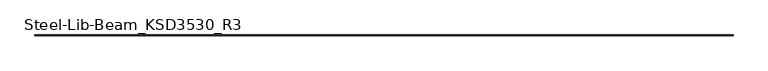
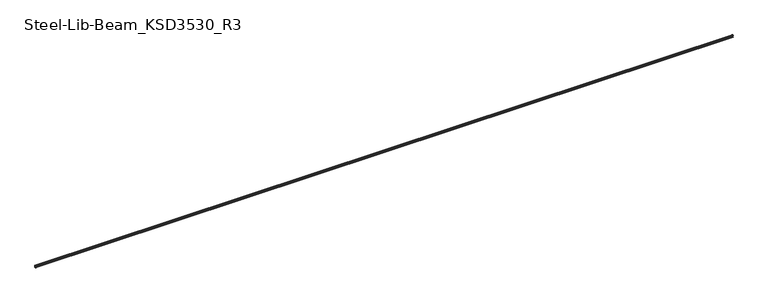
"""IFC4 building model written with IfcOpenShell, lengths in millimetres: beam geometry, Steel-Lib-Beam_KSD3530_R3 : BMS291_C-150×75x20x4.5."""

from ifc_helpers import new_model, si_unit, point, frame, frame_2d, origin, place, context, project, spatial, polyline, circle_curve, trimmed, segment, composite_curve, outline, extrude, source, transform, mapped, element, save


def steel_lib_beam_ksd3530_r3_59e2e9b3(model_context):
    return source(origin(), model_context, "Body", "SweptSolid", [
        extrude(outline(composite_curve([segment(trimmed(circle_curve(frame_2d((-41.0, 66.0)), 9.0), [point((-50.0, 66.0))], [point((-41.0, 75.0))], False, "CARTESIAN"), True, "CONTINUOUS"), segment(polyline([(-41.0, 75.0), (16.0, 75.0)]), True, "CONTINUOUS"), segment(trimmed(circle_curve(frame_2d((16.0, 66.0)), 9.0), [point((16.0, 75.0))], [point((25.0, 66.0))], False, "CARTESIAN"), True, "CONTINUOUS"), segment(polyline([(25.0, 66.0), (25.0, -66.0)]), True, "CONTINUOUS"), segment(trimmed(circle_curve(frame_2d((16.0, -66.0)), 9.0), [point((25.0, -66.0))], [point((16.0, -75.0))], False, "CARTESIAN"), True, "CONTINUOUS"), segment(polyline([(16.0, -75.0), (-41.0, -75.0)]), True, "CONTINUOUS"), segment(trimmed(circle_curve(frame_2d((-41.0, -66.0)), 9.0), [point((-41.0, -75.0))], [point((-50.0, -66.0))], False, "CARTESIAN"), True, "CONTINUOUS"), segment(polyline([(-50.0, -66.0), (-50.0, -55.0), (-45.5, -55.0), (-45.5, -66.0)]), True, "CONTINUOUS"), segment(trimmed(circle_curve(frame_2d((-41.0, -66.0)), 4.5), [point((-45.5, -66.0))], [point((-41.0, -70.5))], True, "CARTESIAN"), True, "CONTINUOUS"), segment(polyline([(-41.0, -70.5), (16.0, -70.5)]), True, "CONTINUOUS"), segment(trimmed(circle_curve(frame_2d((16.0, -66.0)), 4.5), [point((16.0, -70.5))], [point((20.5, -66.0))], True, "CARTESIAN"), True, "CONTINUOUS"), segment(polyline([(20.5, -66.0), (20.5, 66.0)]), True, "CONTINUOUS"), segment(trimmed(circle_curve(frame_2d((16.0, 66.0)), 4.5), [point((20.5, 66.0))], [point((16.0, 70.5))], True, "CARTESIAN"), True, "CONTINUOUS"), segment(polyline([(16.0, 70.5), (-41.0, 70.5)]), True, "CONTINUOUS"), segment(trimmed(circle_curve(frame_2d((-41.0, 66.0)), 4.5), [point((-41.0, 70.5))], [point((-45.5, 66.0))], True, "CARTESIAN"), True, "CONTINUOUS"), segment(polyline([(-45.5, 66.0), (-45.5, 55.0), (-50.0, 55.0), (-50.0, 66.0)]), True, "CONTINUOUS")], self_intersect=False)), frame((-25622.5, 0.0, 0.0), z_axis=(1.0, 0.0, 0.0), x_axis=(0.0, 1.0, 0.0)), (0.0, 0.0, 1.0), 51245.0),
    ])


if __name__ == "__main__":
    model = new_model("IFC4")
    model_context = context("Model", 3, world=origin())
    ifc_project = project(units=[si_unit("LENGTHUNIT", "METRE", prefix="MILLI")], contexts=[model_context])
    site = spatial("IfcSite", under=ifc_project)
    building = spatial("IfcBuilding", under=site)
    placement = place(None, origin())
    steel_lib_beam_ksd3530_r3_shape = steel_lib_beam_ksd3530_r3_59e2e9b3(model_context)
    element("IfcBeam", 1, ObjectType="Steel-Lib-Beam_KSD3530_R3 : BMS291_C-150×75x20x4.5", at=placement, inside=building, context=model_context, shape_type="MappedRepresentation", body=[
        mapped(steel_lib_beam_ksd3530_r3_shape, transform((0.0, 0.0, 0.0), x_axis=(1.0, 0.0, 0.0), y_axis=(0.0, 1.0, 0.0), z_axis=(0.0, 0.0, 1.0))),
    ])
    save(model, "model.ifc")

# Revit data of these elements
# Type "Steel-Lib-Beam_KSD3530_R3 : BMS291_C-150×75x20x4.5"
#   Keynote = "C-150×75x20x4.5"
#   SteelWeight = "Light"
#   x = 0.0250 m
#   t1 = 0.0090 m
#   t = 0.0045 m
#   Surface Area = 0.629834 m²/m
#   Section Area = 13.9688 cm²
#   Mass per Unit Length = 10.9655 kg/m
#   C = 0.0200 m
#   A = 0.0750 m
#   Length [instance default] = 1.5000 m
#   H = 0.1500 m
#   hec_material4 [instance default] = none
#   hec_material3 [instance default] = none
#   hec_material2 [instance default] = none
#   hec_material1 [instance default] = none
#   Structural Material [instance default] = Metal - Steel - Light Gauge
#   Assembly Code = ""
# Element 1 (IfcBeam, "Steel-Lib-Beam_KSD3530_R3 : BMS291_C-150×75x20x4.5")
#   Structural Material = none
# Materials
#   "Metal - Steel - Light Gauge": class "Metal", colour RGB 247 247 247, transparency 0
